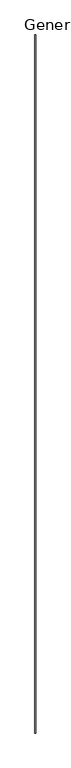
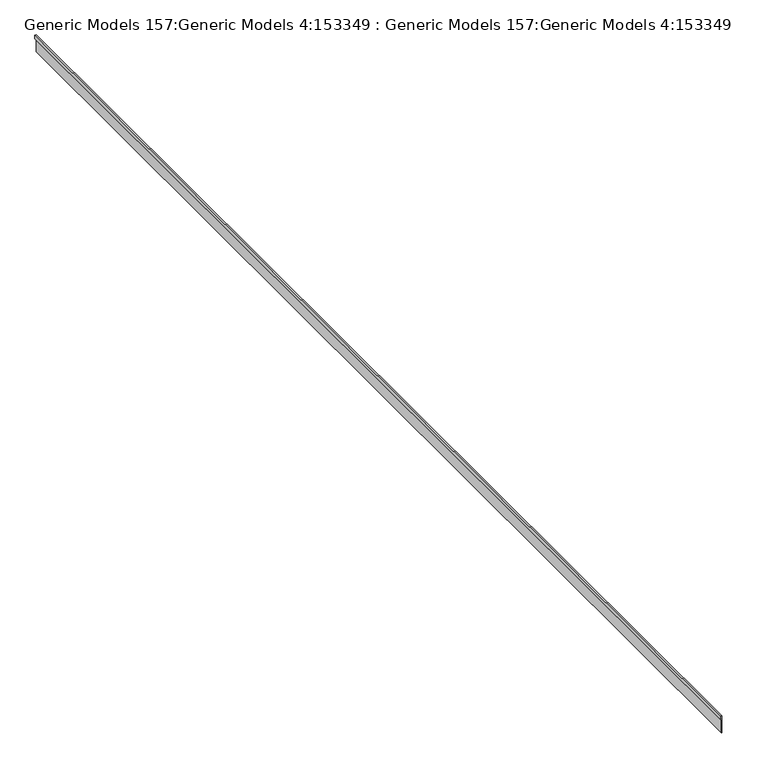
"""IFC4 building model written with IfcOpenShell, lengths in millimetres: proxy geometry, Generic Models 157:Generic Models 4:153349 : Generic Models 157:Generic Models 4:153349."""

import ifcopenshell
import ifcopenshell.guid

model = None  # the IFC model being written
_history = None  # IfcOwnerHistory: only IFC2X3 demands one
_inside = {}  # id of a spatial element -> (the spatial element, [elements in it])
_under = {}  # id of a project, library or spatial element -> (it, [spatial elements below it])
_declared = {}  # id of a project -> (the project, [libraries it declares])
_typed = {}  # id of a type object -> (the type object, [elements of that type])
_made_of = {}  # id of a material, layer set ... -> (it, [elements and type objects made of it])


def new_model(schema):
    """Start an empty IFC model of exactly this schema.

    Asked for "IFC4X3", IfcOpenShell would pick the latest addendum, in which some entities
    have other attributes; the version numbers below select the first issue.
    IFC2X3 requires an IfcOwnerHistory on every rooted entity: one is made here for all.
    """
    global model, _history
    if schema == "IFC4X3":
        model = ifcopenshell.file(schema_version=(4, 3, 0, 0))
    else:
        model = ifcopenshell.file(schema=schema)
    _inside.clear()
    _under.clear()
    _declared.clear()
    _typed.clear()
    _made_of.clear()
    _history = None
    if model.schema == "IFC2X3":
        org = make("IfcOrganization", Name="unknown")
        user = make(
            "IfcPersonAndOrganization",
            ThePerson=make("IfcPerson", FamilyName="unknown"),
            TheOrganization=org,
        )
        app = make(
            "IfcApplication",
            ApplicationDeveloper=org,
            Version="unknown",
            ApplicationFullName="unknown",
            ApplicationIdentifier="unknown",
        )
        _history = make(
            "IfcOwnerHistory",
            OwningUser=user,
            OwningApplication=app,
            ChangeAction="ADDED",
            CreationDate=0,
        )
    return model


def make(cls, **values):
    """One entity of the class cls with the attributes given. An attribute that is None is left unset."""
    return model.create_entity(
        cls, **{name: value for name, value in values.items() if value is not None}
    )


def rooted(cls, **values):
    """An entity with a GlobalId (a new one), such as an element, a storey or a relation."""
    return make(cls, GlobalId=ifcopenshell.guid.new(), OwnerHistory=_history, **values)


def si_unit(unit_type, name, prefix=None):
    """IfcSIUnit, for example si_unit("LENGTHUNIT", "METRE", prefix="MILLI")."""
    return make("IfcSIUnit", UnitType=unit_type, Prefix=prefix, Name=name)


def assignment(units):
    """IfcUnitAssignment: the units of a project."""
    return None if units is None else make("IfcUnitAssignment", Units=units)


def point(xyz):
    """IfcCartesianPoint."""
    return None if xyz is None else make("IfcCartesianPoint", Coordinates=xyz)


def direction(xyz):
    """IfcDirection."""
    return None if xyz is None else make("IfcDirection", DirectionRatios=xyz)


def frame(location, z_axis=None, x_axis=None):
    """IfcAxis2Placement3D, a coordinate frame: its origin and axes. An axis left out is left unset."""
    return make(
        "IfcAxis2Placement3D",
        Location=point(location),
        Axis=direction(z_axis),
        RefDirection=direction(x_axis),
    )


def origin():
    """The frame at (0, 0, 0) with its axes left unset."""
    return frame((0.0, 0.0, 0.0))


def place(relative_to, where):
    """IfcLocalPlacement: puts the frame where relative to a parent placement (None: the world)."""
    return make(
        "IfcLocalPlacement", PlacementRelTo=relative_to, RelativePlacement=where
    )


def context(
    kind, dimensions, precision=None, world=None, true_north=None, identifier=None
):
    """IfcGeometricRepresentationContext, for example the 3D "Model" context."""
    return make(
        "IfcGeometricRepresentationContext",
        ContextIdentifier=identifier,
        ContextType=kind,
        CoordinateSpaceDimension=dimensions,
        Precision=precision,
        WorldCoordinateSystem=world,
        TrueNorth=true_north,
    )


def project(units=None, contexts=None):
    """IfcProject with its units and contexts."""
    return rooted(
        "IfcProject",
        Name="project",
        RepresentationContexts=contexts,
        UnitsInContext=assignment(units),
    )


def spatial(cls, under=None, at=None, **own):
    """A site, building, storey or space (cls), placed at a placement, below another one or the project."""
    s = rooted(cls, ObjectPlacement=at, **own)
    if under is not None:
        _under.setdefault(under.id(), (under, []))[1].append(s)
    return s


def polyline(points):
    """IfcPolyline through the points."""
    return make("IfcPolyline", Points=[point(p) for p in points])


def outline(outer, holes=None, kind="AREA"):
    """IfcArbitraryClosedProfileDef: a profile drawn as a closed curve; with holes, ...WithVoids."""
    if holes is None:
        return make("IfcArbitraryClosedProfileDef", ProfileType=kind, OuterCurve=outer)
    return make(
        "IfcArbitraryProfileDefWithVoids",
        ProfileType=kind,
        OuterCurve=outer,
        InnerCurves=holes,
    )


def extrude(swept, where, along, depth):
    """IfcExtrudedAreaSolid: the profile swept, set in the frame where, extruded along a direction by depth."""
    return make(
        "IfcExtrudedAreaSolid",
        SweptArea=swept,
        Position=where,
        ExtrudedDirection=direction(along),
        Depth=depth,
    )


def shape(context_of_items, identifier, shape_type, items):
    """IfcShapeRepresentation: the items that make up one representation, for example the "Body"."""
    return make(
        "IfcShapeRepresentation",
        ContextOfItems=context_of_items,
        RepresentationIdentifier=identifier,
        RepresentationType=shape_type,
        Items=items,
    )


def source(mapping_origin, context_of_items, identifier, shape_type, items):
    """IfcRepresentationMap: a shape defined once, which mapped items show again and again."""
    return make(
        "IfcRepresentationMap",
        MappingOrigin=mapping_origin,
        MappedRepresentation=shape(context_of_items, identifier, shape_type, items),
    )


def transform(
    local_origin,
    x_axis=None,
    y_axis=None,
    z_axis=None,
    scale=None,
    scale2=None,
    scale3=None,
    uniform=True,
):
    """IfcCartesianTransformationOperator3D, or its non-uniform kind. x_axis, y_axis, z_axis: its Axis1, 2, 3."""
    if uniform:
        return make(
            "IfcCartesianTransformationOperator3D",
            Axis1=direction(x_axis),
            Axis2=direction(y_axis),
            LocalOrigin=point(local_origin),
            Scale=scale,
            Axis3=direction(z_axis),
        )
    return make(
        "IfcCartesianTransformationOperator3DnonUniform",
        Axis1=direction(x_axis),
        Axis2=direction(y_axis),
        LocalOrigin=point(local_origin),
        Scale=scale,
        Axis3=direction(z_axis),
        Scale2=scale2,
        Scale3=scale3,
    )


def mapped(mapping_source, mapping_target):
    """IfcMappedItem: shows the shape of a source again, moved by a transform."""
    return make(
        "IfcMappedItem", MappingSource=mapping_source, MappingTarget=mapping_target
    )


def made_of(thing, what):
    """Note that an element or type object is made of a material, layer set ...; save() writes the relation."""
    if what is not None:
        _made_of.setdefault(what.id(), (what, []))[1].append(thing)
    return thing


def element(
    cls,
    number,
    at=None,
    inside=None,
    cuts=None,
    type_object=None,
    material=None,
    context=None,
    identifier="Body",
    shape_type=None,
    held_by="IfcProductDefinitionShape",
    body=None,
    shapes=None,
    **own,
):
    """One element of the class cls, such as IfcWall. Its Tag is "e" and its number.

    at: its placement. inside: the storey or other place that contains it. cuts: it is an
    opening in that element (IfcRelVoidsElement). A single representation is given by context,
    identifier, shape_type and body (its items); several are given by shapes. held_by: the class
    of the entity that holds the representations. save() writes the other relations.
    """
    e = rooted(cls, Tag="e%d" % number, ObjectPlacement=at, **own)
    if body is not None:
        shapes = [shape(context, identifier, shape_type, body)]
    if shapes is not None:
        e.Representation = make(held_by, Representations=shapes)
    if inside is not None:
        _inside.setdefault(inside.id(), (inside, []))[1].append(e)
    if cuts is not None:
        rooted(
            "IfcRelVoidsElement", RelatingBuildingElement=cuts, RelatedOpeningElement=e
        )
    if type_object is not None:
        _typed.setdefault(type_object.id(), (type_object, []))[1].append(e)
    return made_of(e, material)


def aggregate(whole, parts):
    """IfcRelAggregates: a whole, such as a stair, and the parts it consists of."""
    return rooted("IfcRelAggregates", RelatingObject=whole, RelatedObjects=parts)


def save(model, path):
    """Write the relations noted so far, then the file.

    IfcRelAggregates (storeys below a building ...), IfcRelContainedInSpatialStructure (elements
    in a storey), IfcRelDefinesByType, IfcRelAssociatesMaterial and IfcRelDeclares: one each for
    every whole, place, type object, material and project.
    """
    for whole, parts in _under.values():
        aggregate(whole, parts)
    for where, things in _inside.values():
        rooted(
            "IfcRelContainedInSpatialStructure",
            RelatedElements=things,
            RelatingStructure=where,
        )
    for kind, things in _typed.values():
        rooted("IfcRelDefinesByType", RelatedObjects=things, RelatingType=kind)
    for what, things in _made_of.values():
        rooted("IfcRelAssociatesMaterial", RelatedObjects=things, RelatingMaterial=what)
    for by, libraries in _declared.values():
        rooted("IfcRelDeclares", RelatingContext=by, RelatedDefinitions=libraries)
    model.write(path)


def generic_models_157_generic_models_4_153349_generic_models_b6bb8373(model_context):
    return source(origin(), model_context, "Body", "SweptSolid", [
        extrude(outline(polyline([(-665.8975126, -10280.5078813), (-665.8975126, -10277.3328813), (-503.9725126, -10277.3328813), (-503.9725126, -10278.9203813), (-476.8710353, -10278.9203813), (-476.8710353, -10294.1571126), (-513.4975126, -10294.1571126), (-513.4975126, -10280.5078813), (-665.8975126, -10280.5078813)])), frame((0.0, -5303.1974793, 0.0), z_axis=(0.0, 1.0, 0.0), x_axis=(0.0, 0.0, 1.0)), (0.0, 0.0, 1.0), 12547.6),
    ])


if __name__ == "__main__":
    model = new_model("IFC4")
    model_context = context("Model", 3, world=origin())
    ifc_project = project(units=[si_unit("LENGTHUNIT", "METRE", prefix="MILLI")], contexts=[model_context])
    site = spatial("IfcSite", under=ifc_project)
    building = spatial("IfcBuilding", under=site)
    placement = place(None, origin())
    generic_models_157_generic_models_4_153349_generic_models_shape = generic_models_157_generic_models_4_153349_generic_models_b6bb8373(model_context)
    element("IfcBuildingElementProxy", 1, Name="Generic Models 157:Generic Models 4:153349 : Generic Models 157:Generic Models 4:153349", ObjectType="Generic Models 157:Generic Models 4:153349 : Generic Models 157:Generic Models 4:153349", at=placement, inside=building, context=model_context, shape_type="MappedRepresentation", body=[
        mapped(generic_models_157_generic_models_4_153349_generic_models_shape, transform((0.0, 0.0, 0.0), x_axis=(1.0, 0.0, 0.0), y_axis=(0.0, 1.0, 0.0), z_axis=(0.0, 0.0, 1.0))),
    ])
    save(model, "model.ifc")

# Revit data of these elements
# Type "Generic Models 157:Generic Models 4:153349 : Generic Models 157:Generic Models 4:153349"
#   NameOverride = "Generic Models 157:Generic Models 4:153349"
#   ObjectTypeOverride = "Generic Models 157:Generic Models 4"
#   Reference = "Generic Models 4"
#   Category = "Generic Models"
#   Tag = "153349"
# Element 1 (IfcBuildingElementProxy, "Generic Models 157:Generic Models 4:153349 : Generic Models 157:Generic Models 4:153349")
#   Materials on its faces: "_MORTAR SETTING BED 12838"
# Materials
#   "_MORTAR SETTING BED 12838": class "Unassigned", colour RGB 191 191 191, transparency 0
